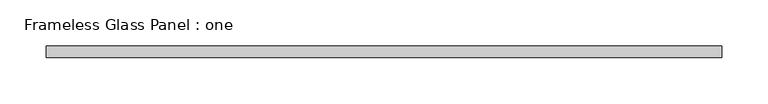
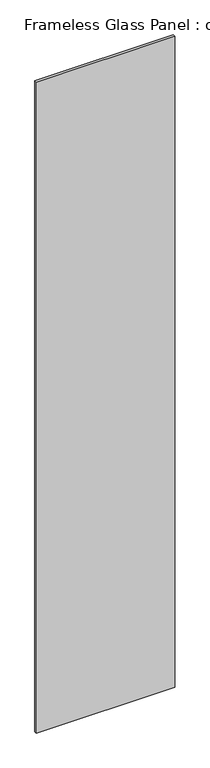
"""IFC4 building model written with IfcOpenShell, lengths in millimetres: plate geometry, Frameless Glass Panel : one."""

from ifc_helpers import new_model, si_unit, origin, origin_with_axes, place, context, project, spatial, polyline, outline, extrude, source, transform, mapped, element, save


def frameless_glass_panel_one_631b8197(model_context):
    return source(origin(), model_context, "Body", "SweptSolid", [
        extrude(outline(polyline([(367.2498217, -6.35), (-367.2498217, -6.35), (-367.2498217, 6.35), (367.2498217, 6.35), (367.2498217, -6.35)])), origin_with_axes(), (0.0, 0.0, 1.0), 3651.25),
    ])


if __name__ == "__main__":
    model = new_model("IFC4")
    model_context = context("Model", 3, world=origin())
    ifc_project = project(units=[si_unit("LENGTHUNIT", "METRE", prefix="MILLI")], contexts=[model_context])
    site = spatial("IfcSite", under=ifc_project)
    building = spatial("IfcBuilding", under=site)
    placement = place(None, origin())
    frameless_glass_panel_one_shape = frameless_glass_panel_one_631b8197(model_context)
    element("IfcPlate", 1, ObjectType="Frameless Glass Panel : one", at=placement, inside=building, context=model_context, shape_type="MappedRepresentation", body=[
        mapped(frameless_glass_panel_one_shape, transform((0.0, 0.0, 0.0), x_axis=(1.0, 0.0, 0.0), y_axis=(0.0, 1.0, 0.0), z_axis=(0.0, 0.0, 1.0))),
    ])
    save(model, "model.ifc")

# Revit data of these elements
# Type "Frameless Glass Panel : one"
#   Glass Thickness = 0' - 0 1/2"
#   Gap btwn Panels = 0' - 0 1/4"
#   Panel Material = TEMPERED GLASS DOOR/SIDELIGHT TO MATCH EXISTING CONF. ROOM
# Element 1 (IfcPlate, "Frameless Glass Panel : one")
#   Materials on its faces: "TEMPERED GLASS DOOR/SIDELIGHT TO MATCH EXISTING CONF. ROOM"
# Materials
#   "TEMPERED GLASS DOOR/SIDELIGHT TO MATCH EXISTING CONF. ROOM": class "Glass", colour RGB 218 227 224, transparency 0.85, Description = "Soda Lime Glass", Cost = 0
